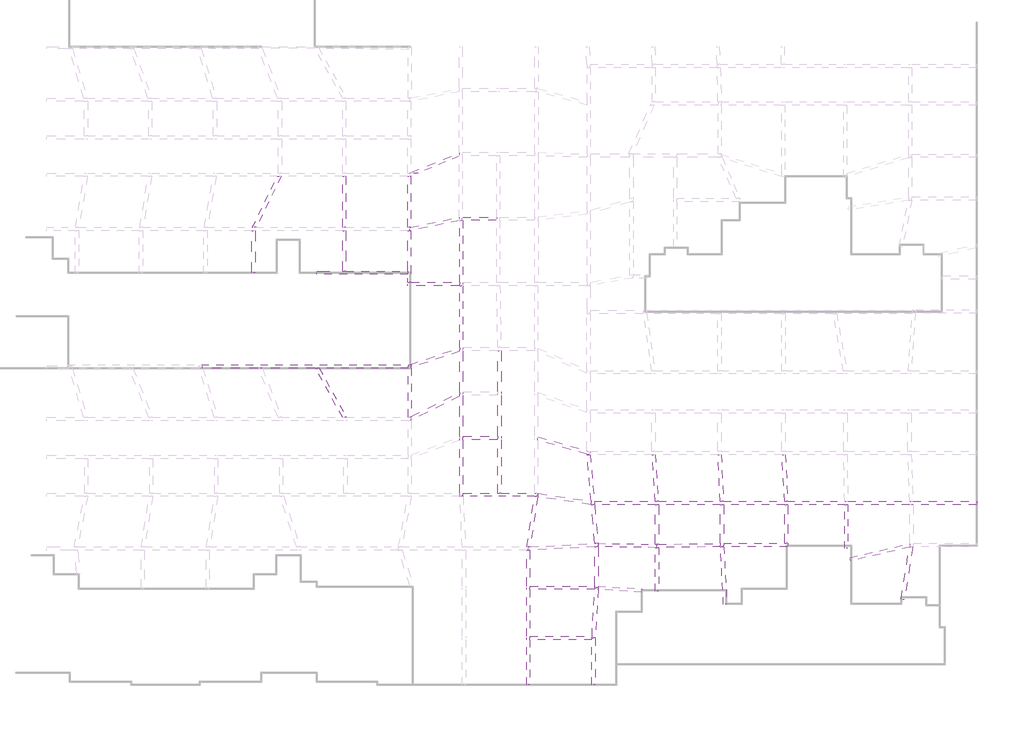
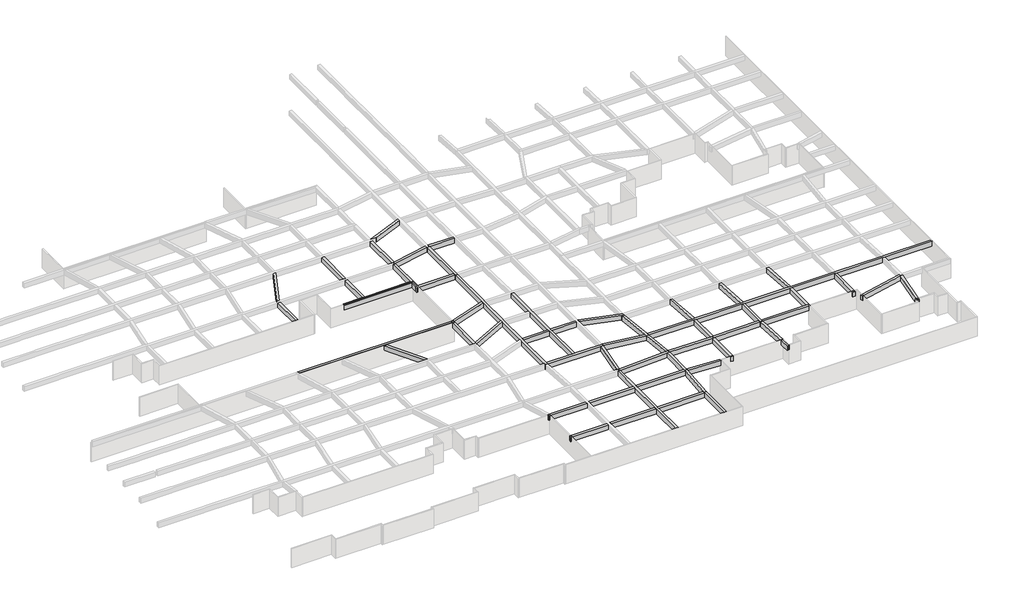
# One storey, part 12 of 45: 49 beams.
"""IFC4 building model written with IfcOpenShell, lengths in millimetres."""

import ifcopenshell
import ifcopenshell.guid

model = None  # the IFC model being written
_history = None  # IfcOwnerHistory: only IFC2X3 demands one
_inside = {}  # id of a spatial element -> (the spatial element, [elements in it])
_under = {}  # id of a project, library or spatial element -> (it, [spatial elements below it])
_declared = {}  # id of a project -> (the project, [libraries it declares])
_typed = {}  # id of a type object -> (the type object, [elements of that type])
_made_of = {}  # id of a material, layer set ... -> (it, [elements and type objects made of it])


def new_model(schema):
    """Start an empty IFC model of exactly this schema.

    Asked for "IFC4X3", IfcOpenShell would pick the latest addendum, in which some entities
    have other attributes; the version numbers below select the first issue.
    IFC2X3 requires an IfcOwnerHistory on every rooted entity: one is made here for all.
    """
    global model, _history
    if schema == "IFC4X3":
        model = ifcopenshell.file(schema_version=(4, 3, 0, 0))
    else:
        model = ifcopenshell.file(schema=schema)
    _inside.clear()
    _under.clear()
    _declared.clear()
    _typed.clear()
    _made_of.clear()
    _history = None
    if model.schema == "IFC2X3":
        org = make("IfcOrganization", Name="unknown")
        user = make(
            "IfcPersonAndOrganization",
            ThePerson=make("IfcPerson", FamilyName="unknown"),
            TheOrganization=org,
        )
        app = make(
            "IfcApplication",
            ApplicationDeveloper=org,
            Version="unknown",
            ApplicationFullName="unknown",
            ApplicationIdentifier="unknown",
        )
        _history = make(
            "IfcOwnerHistory",
            OwningUser=user,
            OwningApplication=app,
            ChangeAction="ADDED",
            CreationDate=0,
        )
    return model


def make(cls, **values):
    """One entity of the class cls with the attributes given. An attribute that is None is left unset."""
    return model.create_entity(
        cls, **{name: value for name, value in values.items() if value is not None}
    )


def rooted(cls, **values):
    """An entity with a GlobalId (a new one), such as an element, a storey or a relation."""
    return make(cls, GlobalId=ifcopenshell.guid.new(), OwnerHistory=_history, **values)


def si_unit(unit_type, name, prefix=None):
    """IfcSIUnit, for example si_unit("LENGTHUNIT", "METRE", prefix="MILLI")."""
    return make("IfcSIUnit", UnitType=unit_type, Prefix=prefix, Name=name)


def assignment(units):
    """IfcUnitAssignment: the units of a project."""
    return None if units is None else make("IfcUnitAssignment", Units=units)


def point(xyz):
    """IfcCartesianPoint."""
    return None if xyz is None else make("IfcCartesianPoint", Coordinates=xyz)


def direction(xyz):
    """IfcDirection."""
    return None if xyz is None else make("IfcDirection", DirectionRatios=xyz)


def frame(location, z_axis=None, x_axis=None):
    """IfcAxis2Placement3D, a coordinate frame: its origin and axes. An axis left out is left unset."""
    return make(
        "IfcAxis2Placement3D",
        Location=point(location),
        Axis=direction(z_axis),
        RefDirection=direction(x_axis),
    )


def origin():
    """The frame at (0, 0, 0) with its axes left unset."""
    return frame((0.0, 0.0, 0.0))


def place(relative_to, where):
    """IfcLocalPlacement: puts the frame where relative to a parent placement (None: the world)."""
    return make(
        "IfcLocalPlacement", PlacementRelTo=relative_to, RelativePlacement=where
    )


def context(
    kind, dimensions, precision=None, world=None, true_north=None, identifier=None
):
    """IfcGeometricRepresentationContext, for example the 3D "Model" context."""
    return make(
        "IfcGeometricRepresentationContext",
        ContextIdentifier=identifier,
        ContextType=kind,
        CoordinateSpaceDimension=dimensions,
        Precision=precision,
        WorldCoordinateSystem=world,
        TrueNorth=true_north,
    )


def project(units=None, contexts=None):
    """IfcProject with its units and contexts."""
    return rooted(
        "IfcProject",
        Name="project",
        RepresentationContexts=contexts,
        UnitsInContext=assignment(units),
    )


def spatial(cls, under=None, at=None, **own):
    """A site, building, storey or space (cls), placed at a placement, below another one or the project."""
    s = rooted(cls, ObjectPlacement=at, **own)
    if under is not None:
        _under.setdefault(under.id(), (under, []))[1].append(s)
    return s


def polyline(points):
    """IfcPolyline through the points."""
    return make("IfcPolyline", Points=[point(p) for p in points])


def outline(outer, holes=None, kind="AREA"):
    """IfcArbitraryClosedProfileDef: a profile drawn as a closed curve; with holes, ...WithVoids."""
    if holes is None:
        return make("IfcArbitraryClosedProfileDef", ProfileType=kind, OuterCurve=outer)
    return make(
        "IfcArbitraryProfileDefWithVoids",
        ProfileType=kind,
        OuterCurve=outer,
        InnerCurves=holes,
    )


def extrude(swept, where, along, depth):
    """IfcExtrudedAreaSolid: the profile swept, set in the frame where, extruded along a direction by depth."""
    return make(
        "IfcExtrudedAreaSolid",
        SweptArea=swept,
        Position=where,
        ExtrudedDirection=direction(along),
        Depth=depth,
    )


def faces_of(points, faces, orient=None, outer=None):
    """IfcFace entities. A face is a list of loops; a loop is a list of indices into points, from 0.

    orient and outer hold one flag for each loop. By default every Orientation is true, the
    first loop of a face is its IfcFaceOuterBound and the others are IfcFaceBound.
    """
    made = []
    for i, loops in enumerate(faces):
        bounds = []
        for j, loop in enumerate(loops):
            is_outer = j == 0 if outer is None else outer[i][j]
            bounds.append(
                make(
                    "IfcFaceOuterBound" if is_outer else "IfcFaceBound",
                    Bound=make("IfcPolyLoop", Polygon=[points[k] for k in loop]),
                    Orientation=True if orient is None else orient[i][j],
                )
            )
        made.append(make("IfcFace", Bounds=bounds))
    return made


def faceted_brep(points, faces, orient=None, outer=None, voids=None):
    """IfcFacetedBrep: a solid bounded by flat faces; with voids (closed shells), ...WithVoids."""
    shared = [point(p) for p in points]
    hull = make("IfcClosedShell", CfsFaces=faces_of(shared, faces, orient, outer))
    if voids is None:
        return make("IfcFacetedBrep", Outer=hull)
    return make(
        "IfcFacetedBrepWithVoids",
        Outer=hull,
        Voids=[
            make(cls, CfsFaces=faces_of(shared, fs, o, b)) for cls, fs, o, b in voids
        ],
    )


def shape(context_of_items, identifier, shape_type, items):
    """IfcShapeRepresentation: the items that make up one representation, for example the "Body"."""
    return make(
        "IfcShapeRepresentation",
        ContextOfItems=context_of_items,
        RepresentationIdentifier=identifier,
        RepresentationType=shape_type,
        Items=items,
    )


def made_of(thing, what):
    """Note that an element or type object is made of a material, layer set ...; save() writes the relation."""
    if what is not None:
        _made_of.setdefault(what.id(), (what, []))[1].append(thing)
    return thing


def element(
    cls,
    number,
    at=None,
    inside=None,
    cuts=None,
    type_object=None,
    material=None,
    context=None,
    identifier="Body",
    shape_type=None,
    held_by="IfcProductDefinitionShape",
    body=None,
    shapes=None,
    **own,
):
    """One element of the class cls, such as IfcWall. Its Tag is "e" and its number.

    at: its placement. inside: the storey or other place that contains it. cuts: it is an
    opening in that element (IfcRelVoidsElement). A single representation is given by context,
    identifier, shape_type and body (its items); several are given by shapes. held_by: the class
    of the entity that holds the representations. save() writes the other relations.
    """
    e = rooted(cls, Tag="e%d" % number, ObjectPlacement=at, **own)
    if body is not None:
        shapes = [shape(context, identifier, shape_type, body)]
    if shapes is not None:
        e.Representation = make(held_by, Representations=shapes)
    if inside is not None:
        _inside.setdefault(inside.id(), (inside, []))[1].append(e)
    if cuts is not None:
        rooted(
            "IfcRelVoidsElement", RelatingBuildingElement=cuts, RelatedOpeningElement=e
        )
    if type_object is not None:
        _typed.setdefault(type_object.id(), (type_object, []))[1].append(e)
    return made_of(e, material)


def aggregate(whole, parts):
    """IfcRelAggregates: a whole, such as a stair, and the parts it consists of."""
    return rooted("IfcRelAggregates", RelatingObject=whole, RelatedObjects=parts)


def save(model, path):
    """Write the relations noted so far, then the file.

    IfcRelAggregates (storeys below a building ...), IfcRelContainedInSpatialStructure (elements
    in a storey), IfcRelDefinesByType, IfcRelAssociatesMaterial and IfcRelDeclares: one each for
    every whole, place, type object, material and project.
    """
    for whole, parts in _under.values():
        aggregate(whole, parts)
    for where, things in _inside.values():
        rooted(
            "IfcRelContainedInSpatialStructure",
            RelatedElements=things,
            RelatingStructure=where,
        )
    for kind, things in _typed.values():
        rooted("IfcRelDefinesByType", RelatedObjects=things, RelatingType=kind)
    for what, things in _made_of.values():
        rooted("IfcRelAssociatesMaterial", RelatedObjects=things, RelatingMaterial=what)
    for by, libraries in _declared.values():
        rooted("IfcRelDeclares", RelatingContext=by, RelatedDefinitions=libraries)
    model.write(path)


model = new_model("IFC4")

# Units and contexts
model_context = context("Model", 3, world=origin())
ifc_project = project(units=[si_unit("LENGTHUNIT", "METRE", prefix="MILLI")], contexts=[model_context])

# Site, building, storey
site = spatial("IfcSite", under=ifc_project)
building = spatial("IfcBuilding", under=site)
storey = spatial("IfcBuildingStorey", under=building, Name="户型图", Elevation=0.0)

# Beams
placement = place(None, origin())
element("IfcBeam", 1, ObjectType="混凝土 - 矩形梁 : KL_beam", at=placement, inside=storey, context=model_context, shape_type="Brep", body=[
    faceted_brep([(-73841.6921627, -136482.7394466, 3300.0), (-73801.0394369, -136882.7394466, 3300.0), (-73674.2267606, -136856.6940178, 3300.0), (-67830.7823984, -135656.5378646, 3300.0), (-67830.7823984, -135248.1884022, 3300.0), (-73674.2267606, -136448.3445554, 3300.0), (-73841.6921627, -136482.7394466, 2500.0), (-67830.7823984, -135248.1884022, 2500.0), (-73674.2267606, -136448.3445554, 2500.0), (-73801.0394369, -136882.7394466, 2500.0), (-67830.7823984, -135656.5378646, 2500.0), (-73674.2267606, -136856.6940178, 2500.0)], [[[0, 1, 2, 3, 4, 5]], [[6, 0, 5, 4, 7, 8]], [[9, 6, 8, 7, 10, 11]], [[1, 9, 11, 10, 3, 2]], [[1, 0, 6, 9]], [[4, 3, 10, 7]]]),
])
element("IfcBeam", 2, ObjectType="混凝土 - 矩形梁 : KL_beam", at=placement, inside=storey, context=model_context, shape_type="Brep", body=[
    faceted_brep([(-73867.4796211, -129869.3244435, 3300.0), (-72799.6927561, -129869.3244435, 3300.0), (-67830.7823984, -127861.7543451, 3300.0), (-67830.7823984, -127430.3404481, 3300.0), (-73674.2267606, -129791.2452196, 3300.0), (-72799.6927561, -129869.3244435, 2500.0), (-67830.7823984, -127861.7543451, 2500.0), (-73867.4796211, -129869.3244435, 2500.0), (-73674.2267606, -129791.2452196, 2500.0), (-67830.7823984, -127430.3404481, 2500.0)], [[[0, 1, 2, 3, 4]], [[1, 5, 6, 2]], [[5, 7, 8, 9, 6]], [[7, 0, 4, 3, 9, 8]], [[1, 0, 7, 5]], [[3, 2, 6, 9]]]),
])
element("IfcBeam", 3, ObjectType="混凝土 - 矩形梁 : KL_beam", at=placement, inside=storey, context=model_context, shape_type="SweptSolid", body=[
    extrude(outline(polyline([(-73841.6921627, -136482.7394466), (-74074.2267606, -136482.7394466), (-74074.2267606, -130269.3244435), (-73789.7274974, -130269.3244435), (-73674.2267606, -130222.6591167), (-73674.2267606, -136448.3445554), (-73841.6921627, -136482.7394466)])), frame((0.0, 0.0, 2500.0), z_axis=(0.0, 0.0, 1.0), x_axis=(1.0, 0.0, 0.0)), (0.0, 0.0, 1.0), 800.0),
])
element("IfcBeam", 4, ObjectType="混凝土 - 矩形梁 : KL_beam", at=placement, inside=storey, context=model_context, shape_type="SweptSolid", body=[
    extrude(outline(polyline([(-81974.2267606, -130269.3244435), (-81574.2267606, -130269.3244435), (-81574.2267606, -136482.7394466), (-81974.2267606, -136482.7394466), (-81974.2267606, -130269.3244435)])), frame((0.0, 0.0, 2500.0), z_axis=(0.0, 0.0, 1.0), x_axis=(1.0, 0.0, 0.0)), (0.0, 0.0, 1.0), 800.0),
])
element("IfcBeam", 5, ObjectType="混凝土 - 矩形梁 : KL_beam", at=placement, inside=storey, context=model_context, shape_type="SweptSolid", body=[
    extrude(outline(polyline([(-89894.2936664, -130269.3244435), (-89449.2528902, -130269.3244435), (-92479.7378735, -136482.7394466), (-92924.7786497, -136482.7394466), (-89894.2936664, -130269.3244435)])), frame((0.0, 0.0, 2500.0), z_axis=(0.0, 0.0, 1.0), x_axis=(1.0, 0.0, 0.0)), (0.0, 0.0, 1.0), 800.0),
])
element("IfcBeam", 6, ObjectType="混凝土 - 矩形梁 : KL_beam", at=placement, inside=storey, context=model_context, shape_type="SweptSolid", body=[
    extrude(outline(polyline([(-92600.0024046, -141982.9420425), (-93000.0024046, -141982.9420425), (-93000.0024046, -136882.7394466), (-92600.0024046, -136882.7394466), (-92600.0024046, -141982.9420425)])), frame((0.0, 0.0, 2500.0), z_axis=(0.0, 0.0, 1.0), x_axis=(1.0, 0.0, 0.0)), (0.0, 0.0, 1.0), 800.0),
])
element("IfcBeam", 7, ObjectType="混凝土 - 矩形梁 : KL_beam", at=placement, inside=storey, context=model_context, shape_type="Brep", body=[
    faceted_brep([(-67430.7823984, -135211.286122, 3300.0), (-67430.7823984, -135574.3838418, 3300.0), (-67610.4560354, -135611.286122, 3300.0), (-67364.0267672, -135611.286122, 3300.0), (-63277.6696197, -135611.286122, 3300.0), (-63277.6696197, -135211.286122, 3300.0), (-67610.4560354, -135611.286122, 2500.0), (-67364.0267672, -135611.286122, 2500.0), (-63277.6696197, -135611.286122, 2500.0), (-67430.7823984, -135574.3838418, 2500.0), (-67430.7823984, -135211.286122, 2500.0), (-63277.6696197, -135211.286122, 2500.0)], [[[0, 1, 2, 3, 4, 5]], [[2, 6, 7, 8, 4, 3]], [[9, 10, 11, 8, 7, 6]], [[10, 0, 5, 11]], [[9, 1, 0, 10]], [[1, 9, 6, 2]], [[5, 4, 8, 11]]]),
])
element("IfcBeam", 8, ObjectType="混凝土 - 矩形梁 : KL_beam", at=placement, inside=storey, context=model_context, shape_type="Brep", body=[
    faceted_brep([(-67764.0267672, -143549.8954633, 3300.0), (-67763.6944245, -143549.8954633, 3300.0), (-67364.0267672, -143549.8954633, 3300.0), (-67364.0267672, -143149.8954633, 3300.0), (-67364.0267672, -135611.286122, 3300.0), (-67610.4560354, -135611.286122, 3300.0), (-67764.0267672, -135642.8272555, 3300.0), (-67764.0267672, -143149.8954633, 3300.0), (-67364.0267672, -143549.8954633, 2500.0), (-67364.0267672, -143149.8954633, 2500.0), (-67364.0267672, -135611.286122, 2500.0), (-67763.6944245, -143549.8954633, 2500.0), (-67764.0267672, -143549.8954633, 2500.0), (-67764.0267672, -143149.8954633, 2500.0), (-67764.0267672, -135642.8272555, 2500.0), (-67610.4560354, -135611.286122, 2500.0)], [[[0, 1, 2, 3, 4, 5, 6, 7]], [[2, 8, 9, 10, 4, 3]], [[8, 11, 12, 13, 14, 15, 10, 9]], [[6, 14, 13, 12, 0, 7]], [[14, 6, 5, 15]], [[5, 4, 10, 15]], [[2, 1, 0, 12, 11, 8]]]),
])
element("IfcBeam", 9, ObjectType="混凝土 - 矩形梁 : KL_beam", at=placement, inside=storey, context=model_context, shape_type="Brep", body=[
    faceted_brep([(-67363.6944245, -143549.8954633, 3300.0), (-67364.0267672, -143549.8954633, 3300.0), (-67763.6944245, -143549.8954633, 3300.0), (-67763.6944245, -151106.0765434, 3300.0), (-67763.6944245, -151528.0229867, 3300.0), (-67763.6944245, -156525.7729118, 3300.0), (-67763.6944245, -156972.1576109, 3300.0), (-67763.6944245, -161910.3096227, 3300.0), (-67763.6944245, -162336.4574801, 3300.0), (-67763.6944245, -168748.040132, 3300.0), (-67763.6944245, -168955.1326476, 3300.0), (-67763.6944245, -169148.040132, 3300.0), (-67763.6944245, -169149.8954633, 3300.0), (-67753.4873378, -169149.8954633, 3300.0), (-67363.6944245, -169149.8954633, 3300.0), (-67363.6944245, -168749.8954633, 3300.0), (-67363.6944245, -162249.8954633, 3300.0), (-67363.6944245, -161849.8954633, 3300.0), (-67363.6944245, -156849.8954633, 3300.0), (-67363.6944245, -156449.8954633, 3300.0), (-67363.6944245, -151449.8954633, 3300.0), (-67363.6944245, -151049.8954633, 3300.0), (-67763.6944245, -143549.8954633, 2500.0), (-67763.6944245, -151106.0765434, 2500.0), (-67763.6944245, -151528.0229867, 2500.0), (-67763.6944245, -156525.7729118, 2500.0), (-67763.6944245, -156972.1576109, 2500.0), (-67763.6944245, -161910.3096227, 2500.0), (-67763.6944245, -162336.4574801, 2500.0), (-67763.6944245, -168748.040132, 2500.0), (-67763.6944245, -168955.1326476, 2500.0), (-67763.6944245, -169148.040132, 2500.0), (-67763.6944245, -169149.8954633, 2500.0), (-67364.0267672, -143549.8954633, 2500.0), (-67363.6944245, -143549.8954633, 2500.0), (-67363.6944245, -151049.8954633, 2500.0), (-67363.6944245, -151449.8954633, 2500.0), (-67363.6944245, -156449.8954633, 2500.0), (-67363.6944245, -156849.8954633, 2500.0), (-67363.6944245, -161849.8954633, 2500.0), (-67363.6944245, -162249.8954633, 2500.0), (-67363.6944245, -168749.8954633, 2500.0), (-67363.6944245, -169149.8954633, 2500.0), (-67753.4873378, -169149.8954633, 2500.0)], [[[0, 1, 2, 3, 4, 5, 6, 7, 8, 9, 10, 11, 12, 13, 14, 15, 16, 17, 18, 19, 20, 21]], [[2, 22, 23, 24, 25, 26, 27, 28, 29, 30, 31, 32, 12, 11, 10, 9, 8, 7, 6, 5, 4, 3]], [[22, 33, 34, 35, 36, 37, 38, 39, 40, 41, 42, 43, 32, 31, 30, 29, 28, 27, 26, 25, 24, 23]], [[14, 42, 41, 40, 39, 38, 37, 36, 35, 34, 0, 21, 20, 19, 18, 17, 16, 15]], [[0, 34, 33, 22, 2, 1]], [[14, 13, 12, 32, 43, 42]]]),
])
element("IfcBeam", 10, ObjectType="混凝土 - 矩形梁 : KL_beam", at=placement, inside=storey, context=model_context, shape_type="Brep", body=[
    faceted_brep([(-58263.6944245, -169149.8954633, 3300.0), (-58263.6944245, -168964.6073199, 3300.0), (-58263.6944245, -168777.3030911, 3300.0), (-58263.6944245, -168749.8954633, 3300.0), (-58663.6944245, -168749.8954633, 3300.0), (-62739.7956089, -168749.8954633, 3300.0), (-63139.7956089, -168749.8954633, 3300.0), (-67363.6944245, -168749.8954633, 3300.0), (-67363.6944245, -169149.8954633, 3300.0), (-67352.9383994, -169149.8954633, 3300.0), (-58695.4543771, -169149.8954633, 3300.0), (-58291.1020523, -169149.8954633, 3300.0), (-58263.6944245, -169149.8954633, 2500.0), (-67363.6944245, -169149.8954633, 2500.0), (-67352.9383994, -169149.8954633, 2500.0), (-58695.4543771, -169149.8954633, 2500.0), (-58291.1020523, -169149.8954633, 2500.0), (-58263.6944245, -168749.8954633, 2500.0), (-58263.6944245, -168777.3030911, 2500.0), (-58263.6944245, -168964.6073199, 2500.0), (-67363.6944245, -168749.8954633, 2500.0), (-63139.7956089, -168749.8954633, 2500.0), (-62739.7956089, -168749.8954633, 2500.0), (-58663.6944245, -168749.8954633, 2500.0)], [[[0, 1, 2, 3, 4, 5, 6, 7, 8, 9, 10, 11]], [[12, 0, 11, 10, 9, 8, 13, 14, 15, 16]], [[17, 18, 19, 12, 16, 15, 14, 13, 20, 21, 22, 23]], [[3, 17, 23, 22, 21, 20, 7, 6, 5, 4]], [[8, 7, 20, 13]], [[3, 2, 1, 0, 12, 19, 18, 17]]]),
])
element("IfcBeam", 11, ObjectType="混凝土 - 矩形梁 : KL_beam", at=placement, inside=storey, context=model_context, shape_type="Brep", body=[
    faceted_brep([(-63139.7956089, -168749.8954633, 2500.0), (-63139.7956089, -168749.8954633, 3300.0), (-63139.7956089, -162249.8954633, 3300.0), (-63139.7956089, -161849.8954633, 3300.0), (-63139.7956089, -156849.8954633, 3300.0), (-63139.7956089, -156449.8954633, 3300.0), (-63139.7956089, -151449.8954633, 3300.0), (-63139.7956089, -151449.8954633, 2500.0), (-63139.7956089, -156449.8954633, 2500.0), (-63139.7956089, -156849.8954633, 2500.0), (-63139.7956089, -161849.8954633, 2500.0), (-63139.7956089, -162249.8954633, 2500.0), (-62739.7956089, -168749.8954633, 3300.0), (-62739.7956089, -168749.8954633, 2500.0), (-62739.7956089, -151449.8954633, 3300.0), (-62739.7956089, -151449.8954633, 2500.0), (-62739.7956089, -162249.8954633, 3300.0), (-62739.7956089, -161849.8954633, 3300.0), (-62739.7956089, -156849.8954633, 3300.0), (-62739.7956089, -156449.8954633, 3300.0), (-62739.7956089, -156449.8954633, 2500.0), (-62739.7956089, -156849.8954633, 2500.0), (-62739.7956089, -161849.8954633, 2500.0), (-62739.7956089, -162249.8954633, 2500.0)], [[[0, 1, 2, 3, 4, 5, 6, 7, 8, 9, 10, 11]], [[12, 1, 0, 13]], [[14, 15, 7, 6]], [[1, 12, 16, 17, 18, 19, 14, 6, 5, 4, 3, 2]], [[13, 0, 11, 10, 9, 8, 7, 15, 20, 21, 22, 23]], [[12, 13, 23, 22, 21, 20, 15, 14, 19, 18, 17, 16]]]),
])
element("IfcBeam", 12, ObjectType="混凝土 - 矩形梁 : KL_beam", at=placement, inside=storey, context=model_context, shape_type="Brep", body=[
    faceted_brep([(-52029.6221736, -164102.89588, 3300.0), (-52020.0590892, -164069.5454413, 3300.0), (-51919.3672313, -163718.3912016, 3300.0), (-52319.3672313, -163603.6930473, 3300.0), (-58263.6944245, -161899.1846532, 3300.0), (-58263.6944245, -162315.3044276, 3300.0), (-52306.232201, -164023.579231, 3300.0), (-52145.9289751, -164069.5454413, 3300.0), (-52029.6221736, -164102.89588, 2500.0), (-58263.6944245, -162315.3044276, 2500.0), (-52306.232201, -164023.579231, 2500.0), (-52145.9289751, -164069.5454413, 2500.0), (-51919.3672313, -163718.3912016, 2500.0), (-52020.0590892, -164069.5454413, 2500.0), (-58263.6944245, -161899.1846532, 2500.0), (-52319.3672313, -163603.6930473, 2500.0)], [[[0, 1, 2, 3, 4, 5, 6, 7]], [[8, 0, 7, 6, 5, 9, 10, 11]], [[12, 13, 8, 11, 10, 9, 14, 15]], [[2, 12, 15, 14, 4, 3]], [[5, 4, 14, 9]], [[2, 1, 0, 8, 13, 12]]]),
])
element("IfcBeam", 13, ObjectType="混凝土 - 矩形梁 : KL_beam", at=placement, inside=storey, context=model_context, shape_type="Brep", body=[
    faceted_brep([(-51770.5606479, -170146.3330997, 3300.0), (-51369.0327129, -170146.3330997, 3300.0), (-51404.0281783, -169746.3330997, 3300.0), (-51900.6827437, -164069.5454413, 3300.0), (-51919.3672313, -164069.5454413, 3300.0), (-52020.0590892, -164069.5454413, 3300.0), (-52029.6221736, -164102.89588, 3300.0), (-52145.9289751, -164069.5454413, 3300.0), (-52302.2106787, -164069.5454413, 3300.0), (-51806.7747625, -169732.4038754, 3300.0), (-51770.9347036, -170142.0576241, 3300.0), (-52302.2106787, -164069.5454413, 2500.0), (-51806.7747625, -169732.4038754, 2500.0), (-51770.9347036, -170142.0576241, 2500.0), (-51770.5606479, -170146.3330997, 2500.0), (-51369.0327129, -170146.3330997, 2500.0), (-52145.9289751, -164069.5454413, 2500.0), (-52029.6221736, -164102.89588, 2500.0), (-52020.0590892, -164069.5454413, 2500.0), (-51919.3672313, -164069.5454413, 2500.0), (-51900.6827437, -164069.5454413, 2500.0), (-51404.0281783, -169746.3330997, 2500.0)], [[[0, 1, 2, 3, 4, 5, 6, 7, 8, 9, 10]], [[8, 11, 12, 13, 14, 0, 10, 9]], [[15, 14, 13, 12, 11, 16, 17, 18, 19, 20, 21]], [[20, 3, 2, 1, 15, 21]], [[11, 8, 7, 16]], [[6, 17, 16, 7]], [[17, 6, 5, 18]], [[3, 20, 19, 18, 5, 4]], [[1, 0, 14, 15]]]),
])
element("IfcBeam", 14, ObjectType="混凝土 - 矩形梁 : KL_beam", at=placement, inside=storey, context=model_context, shape_type="Brep", body=[
    faceted_brep([(-4940.9080348, -169746.3330997, 3300.0), (-4940.9080348, -170146.3330997, 3300.0), (-4940.9080348, -170146.3330997, 2500.0), (-4940.9080348, -169746.3330997, 2500.0), (-12714.0233753, -169746.3330997, 3300.0), (-13114.267193, -169746.3330997, 3300.0), (-20616.7570555, -169746.3330997, 3300.0), (-21016.8179867, -169746.3330997, 3300.0), (-27911.1033716, -169746.3330997, 3300.0), (-28311.65231, -169746.3330997, 3300.0), (-35711.0778615, -169746.3330997, 3300.0), (-36111.6267999, -169746.3330997, 3300.0), (-43613.8318582, -169746.3330997, 3300.0), (-44014.7807223, -169746.3330997, 3300.0), (-51404.0281783, -169746.3330997, 3300.0), (-51369.0327129, -170146.3330997, 3300.0), (-44000.5141412, -170146.3330997, 3300.0), (-43600.5141412, -170146.3330997, 3300.0), (-36100.8707749, -170146.3330997, 3300.0), (-35700.8707749, -170146.3330997, 3300.0), (-28300.8996112, -170146.3330997, 3300.0), (-27900.8996112, -170146.3330997, 3300.0), (-21013.2940066, -170146.3330997, 3300.0), (-20613.2940066, -170146.3330997, 3300.0), (-13107.1611302, -170146.3330997, 3300.0), (-12707.1611302, -170146.3330997, 3300.0), (-51369.0327129, -170146.3330997, 2500.0), (-44000.5141412, -170146.3330997, 2500.0), (-43600.5141412, -170146.3330997, 2500.0), (-36100.8707749, -170146.3330997, 2500.0), (-35700.8707749, -170146.3330997, 2500.0), (-28300.8996112, -170146.3330997, 2500.0), (-27900.8996112, -170146.3330997, 2500.0), (-21013.2940066, -170146.3330997, 2500.0), (-20613.2940066, -170146.3330997, 2500.0), (-13107.1611302, -170146.3330997, 2500.0), (-12707.1611302, -170146.3330997, 2500.0), (-51404.0281783, -169746.3330997, 2500.0), (-44014.7807223, -169746.3330997, 2500.0), (-43613.8318582, -169746.3330997, 2500.0), (-36111.6267999, -169746.3330997, 2500.0), (-35711.0778615, -169746.3330997, 2500.0), (-28311.65231, -169746.3330997, 2500.0), (-27911.1033716, -169746.3330997, 2500.0), (-21016.8179867, -169746.3330997, 2500.0), (-20616.7570555, -169746.3330997, 2500.0), (-13114.267193, -169746.3330997, 2500.0), (-12714.0233753, -169746.3330997, 2500.0)], [[[0, 1, 2, 3]], [[1, 0, 4, 5, 6, 7, 8, 9, 10, 11, 12, 13, 14, 15, 16, 17, 18, 19, 20, 21, 22, 23, 24, 25]], [[2, 1, 25, 24, 23, 22, 21, 20, 19, 18, 17, 16, 15, 26, 27, 28, 29, 30, 31, 32, 33, 34, 35, 36]], [[3, 2, 36, 35, 34, 33, 32, 31, 30, 29, 28, 27, 26, 37, 38, 39, 40, 41, 42, 43, 44, 45, 46, 47]], [[0, 3, 47, 46, 45, 44, 43, 42, 41, 40, 39, 38, 37, 14, 13, 12, 11, 10, 9, 8, 7, 6, 5, 4]], [[15, 14, 37, 26]]]),
])
element("IfcBeam", 15, ObjectType="混凝土 - 矩形梁 : KL_beam", at=placement, inside=storey, context=model_context, shape_type="SweptSolid", body=[
    extrude(outline(polyline([(-36409.1346345, -164069.5454413), (-36008.5856961, -164069.5454413), (-35711.0778615, -169746.3330997), (-36111.6267999, -169746.3330997), (-36409.1346345, -164069.5454413)])), frame((0.0, 0.0, 2500.0), z_axis=(0.0, 0.0, 1.0), x_axis=(1.0, 0.0, 0.0)), (0.0, 0.0, 1.0), 800.0),
])
element("IfcBeam", 16, ObjectType="混凝土 - 矩形梁 : KL_beam", at=placement, inside=storey, context=model_context, shape_type="Brep", body=[
    faceted_brep([(-36100.8707749, -175246.3330997, 3300.0), (-35899.5132097, -175246.3330997, 3300.0), (-35700.8707749, -175246.3330997, 3300.0), (-35700.8707749, -174846.3330997, 3300.0), (-35700.8707749, -170146.3330997, 3300.0), (-36100.8707749, -170146.3330997, 3300.0), (-36100.8707749, -174849.0299244, 3300.0), (-36100.8707749, -175246.3330997, 2500.0), (-36100.8707749, -170146.3330997, 2500.0), (-36100.8707749, -174849.0299244, 2500.0), (-35700.8707749, -175246.3330997, 2500.0), (-35899.5132097, -175246.3330997, 2500.0), (-35700.8707749, -170146.3330997, 2500.0), (-35700.8707749, -174846.3330997, 2500.0)], [[[0, 1, 2, 3, 4, 5, 6]], [[7, 0, 6, 5, 8, 9]], [[10, 11, 7, 9, 8, 12, 13]], [[2, 10, 13, 12, 4, 3]], [[5, 4, 12, 8]], [[2, 1, 0, 7, 11, 10]]]),
])
element("IfcBeam", 17, ObjectType="混凝土 - 矩形梁 : KL_beam", at=placement, inside=storey, context=model_context, shape_type="SweptSolid", body=[
    extrude(outline(polyline([(-28609.1601446, -164069.5454413), (-28208.6112062, -164069.5454413), (-27911.1033716, -169746.3330997), (-28311.65231, -169746.3330997), (-28609.1601446, -164069.5454413)])), frame((0.0, 0.0, 2500.0), z_axis=(0.0, 0.0, 1.0), x_axis=(1.0, 0.0, 0.0)), (0.0, 0.0, 1.0), 800.0),
])
element("IfcBeam", 18, ObjectType="混凝土 - 矩形梁 : KL_beam", at=placement, inside=storey, context=model_context, shape_type="Brep", body=[
    faceted_brep([(-27900.8996112, -175246.3330997, 3300.0), (-27900.8996112, -174846.3330997, 3300.0), (-28300.8996112, -174846.3330997, 3300.0), (-35700.8707749, -174846.3330997, 3300.0), (-35700.8707749, -175246.3330997, 3300.0), (-35689.629168, -175246.3330997, 3300.0), (-27900.8996112, -175246.3330997, 2500.0), (-35700.8707749, -175246.3330997, 2500.0), (-35689.629168, -175246.3330997, 2500.0), (-27900.8996112, -174846.3330997, 2500.0), (-35700.8707749, -174846.3330997, 2500.0), (-28300.8996112, -174846.3330997, 2500.0)], [[[0, 1, 2, 3, 4, 5]], [[6, 0, 5, 4, 7, 8]], [[9, 6, 8, 7, 10, 11]], [[1, 9, 11, 10, 3, 2]], [[4, 3, 10, 7]], [[1, 0, 6, 9]]]),
])
element("IfcBeam", 19, ObjectType="混凝土 - 矩形梁 : KL_beam", at=placement, inside=storey, context=model_context, shape_type="SweptSolid", body=[
    extrude(outline(polyline([(-27900.8996112, -174846.3330997), (-28300.8996112, -174846.3330997), (-28300.8996112, -170146.3330997), (-27900.8996112, -170146.3330997), (-27900.8996112, -174846.3330997)])), frame((0.0, 0.0, 2500.0), z_axis=(0.0, 0.0, 1.0), x_axis=(1.0, 0.0, 0.0)), (0.0, 0.0, 1.0), 800.0),
])
element("IfcBeam", 20, ObjectType="混凝土 - 矩形梁 : KL_beam", at=placement, inside=storey, context=model_context, shape_type="SweptSolid", body=[
    extrude(outline(polyline([(-20613.2940066, -175446.4047579), (-21013.2940066, -175446.4047579), (-21013.2940066, -170146.3330997), (-20613.2940066, -170146.3330997), (-20613.2940066, -175446.4047579)])), frame((0.0, 0.0, 2500.0), z_axis=(0.0, 0.0, 1.0), x_axis=(1.0, 0.0, 0.0)), (0.0, 0.0, 1.0), 800.0),
])
element("IfcBeam", 21, ObjectType="混凝土 - 矩形梁 : KL_beam", at=placement, inside=storey, context=model_context, shape_type="Brep", body=[
    faceted_brep([(-43800.2460734, -175353.5956365, 3300.0), (-43600.1428301, -175350.8789795, 3300.0), (-36090.0425443, -175248.9197787, 3300.0), (-35899.5132097, -175246.3330997, 3300.0), (-36100.8707749, -175246.3330997, 3300.0), (-36100.8707749, -174849.0299244, 3300.0), (-43600.5141412, -174950.8471592, 3300.0), (-43800.0395867, -174953.5559719, 3300.0), (-36100.8707749, -174849.0299244, 2500.0), (-43600.5141412, -174950.8471592, 2500.0), (-43800.0395867, -174953.5559719, 2500.0), (-36100.8707749, -175246.3330997, 2500.0), (-35899.5132097, -175246.3330997, 2500.0), (-36090.0425443, -175248.9197787, 2500.0), (-43600.1428301, -175350.8789795, 2500.0), (-43800.2460734, -175353.5956365, 2500.0)], [[[0, 1, 2, 3, 4, 5, 6, 7]], [[7, 6, 5, 8, 9, 10]], [[10, 9, 8, 11, 12, 13, 14, 15]], [[3, 2, 1, 0, 15, 14, 13, 12]], [[4, 11, 8, 5]], [[11, 4, 3, 12]], [[0, 7, 10, 15]]]),
])
element("IfcBeam", 22, ObjectType="混凝土 - 矩形梁 : KL_beam", at=placement, inside=storey, context=model_context, shape_type="Brep", body=[
    faceted_brep([(-59434.9645519, -175280.7215365, 3300.0), (-59424.4901833, -175680.7215365, 3300.0), (-59229.7273676, -175670.5144499, 3300.0), (-51349.1150073, -175257.5090567, 3300.0), (-50949.1150073, -175236.545945, 3300.0), (-50937.7619715, -175235.9509576, 3300.0), (-50949.1150073, -175019.3221294, 3300.0), (-50958.0419428, -174848.9860526, 3300.0), (-50958.696354, -174836.4991437, 3300.0), (-51358.3916515, -174857.4462866, 3300.0), (-59196.1158349, -175268.2040057, 3300.0), (-59434.9645519, -175280.7215365, 2500.0), (-50958.696354, -174836.4991437, 2500.0), (-51358.3916515, -174857.4462866, 2500.0), (-59196.1158349, -175268.2040057, 2500.0), (-59424.4901833, -175680.7215365, 2500.0), (-50958.0419428, -174848.9860526, 2500.0), (-50949.1150073, -175019.3221294, 2500.0), (-50937.7619715, -175235.9509576, 2500.0), (-50949.1150073, -175236.545945, 2500.0), (-51349.1150073, -175257.5090567, 2500.0), (-59229.7273676, -175670.5144499, 2500.0)], [[[0, 1, 2, 3, 4, 5, 6, 7, 8, 9, 10]], [[11, 0, 10, 9, 8, 12, 13, 14]], [[15, 11, 14, 13, 12, 16, 17, 18, 19, 20, 21]], [[1, 15, 21, 20, 19, 18, 5, 4, 3, 2]], [[5, 18, 17, 16, 12, 8, 7, 6]], [[1, 0, 11, 15]]]),
])
element("IfcBeam", 23, ObjectType="混凝土 - 矩形梁 : KL_beam", at=placement, inside=storey, context=model_context, shape_type="Brep", body=[
    faceted_brep([(-59229.7273676, -192027.8669315, 3300.0), (-59629.7273676, -192027.8669315, 3300.0), (-59629.7273676, -192027.8669315, 2500.0), (-59229.7273676, -192027.8669315, 2500.0), (-59229.7273676, -186528.0123265, 3300.0), (-59229.7273676, -186128.0123265, 3300.0), (-59229.7273676, -180443.730522, 3300.0), (-59229.7273676, -180043.730522, 3300.0), (-59229.7273676, -175670.5144499, 3300.0), (-59424.4901833, -175680.7215365, 3300.0), (-59629.7273676, -175680.7215365, 3300.0), (-59629.7273676, -180043.730522, 3300.0), (-59629.7273676, -180443.730522, 3300.0), (-59629.7273676, -186128.0123265, 3300.0), (-59629.7273676, -186528.0123265, 3300.0), (-59629.7273676, -175680.7215365, 2500.0), (-59629.7273676, -180043.730522, 2500.0), (-59629.7273676, -180443.730522, 2500.0), (-59629.7273676, -186128.0123265, 2500.0), (-59629.7273676, -186528.0123265, 2500.0), (-59424.4901833, -175680.7215365, 2500.0), (-59229.7273676, -175670.5144499, 2500.0), (-59229.7273676, -180043.730522, 2500.0), (-59229.7273676, -180443.730522, 2500.0), (-59229.7273676, -186128.0123265, 2500.0), (-59229.7273676, -186528.0123265, 2500.0)], [[[0, 1, 2, 3]], [[1, 0, 4, 5, 6, 7, 8, 9, 10, 11, 12, 13, 14]], [[2, 1, 14, 13, 12, 11, 10, 15, 16, 17, 18, 19]], [[3, 2, 19, 18, 17, 16, 15, 20, 21, 22, 23, 24, 25]], [[0, 3, 25, 24, 23, 22, 21, 8, 7, 6, 5, 4]], [[9, 8, 21, 20]], [[10, 9, 20, 15]]]),
])
element("IfcBeam", 24, ObjectType="混凝土 - 矩形梁 : KL_beam", at=placement, inside=storey, context=model_context, shape_type="Brep", body=[
    faceted_brep([(-51700.5216564, -192028.0123265, 3300.0), (-51700.5216564, -192028.0123265, 2500.0), (-51300.5216564, -192028.0123265, 2500.0), (-51300.5216564, -192028.0123265, 3300.0), (-51300.5216564, -186333.7831438, 3300.0), (-51700.5216564, -186322.2415091, 3300.0), (-51700.5216564, -186528.0123265, 3300.0), (-51300.5216564, -186333.7831438, 2500.0), (-51700.5216564, -186322.2415091, 2500.0), (-51700.5216564, -186528.0123265, 2500.0)], [[[0, 1, 2, 3]], [[4, 5, 6, 0, 3]], [[7, 4, 3, 2]], [[8, 7, 2, 1, 9]], [[5, 8, 9, 1, 0, 6]], [[5, 4, 7, 8]]]),
])
element("IfcBeam", 25, ObjectType="混凝土 - 矩形梁 : KL_beam", at=placement, inside=storey, context=model_context, shape_type="Brep", body=[
    faceted_brep([(-51300.5216564, -186333.7831438, 3300.0), (-50960.9810787, -180454.9298094, 3300.0), (-50949.1150073, -180249.4789789, 3300.0), (-51349.1150073, -180237.9373442, 3300.0), (-51361.0008515, -180443.730522, 3300.0), (-51689.3037054, -186128.0123265, 3300.0), (-51700.5216564, -186322.2415091, 3300.0), (-51349.1150073, -180237.9373442, 2500.0), (-51361.0008515, -180443.730522, 2500.0), (-51689.3037054, -186128.0123265, 2500.0), (-51700.5216564, -186322.2415091, 2500.0), (-50949.1150073, -180249.4789789, 2500.0), (-50960.9810787, -180454.9298094, 2500.0), (-51300.5216564, -186333.7831438, 2500.0)], [[[0, 1, 2, 3, 4, 5, 6]], [[6, 5, 4, 3, 7, 8, 9, 10]], [[10, 9, 8, 7, 11, 12, 13]], [[2, 1, 0, 13, 12, 11]], [[0, 6, 10, 13]], [[2, 11, 7, 3]]]),
])
element("IfcBeam", 26, ObjectType="混凝土 - 矩形梁 : KL_beam", at=placement, inside=storey, context=model_context, shape_type="Brep", body=[
    faceted_brep([(-50949.1150073, -174849.1164646, 3300.0), (-50957.6033304, -174848.9924602, 3300.0), (-50958.0419428, -174848.9860526, 3300.0), (-50949.1150073, -175019.3221294, 3300.0), (-50949.1150073, -174946.0144374, 3300.0), (-50949.1150073, -174849.1164646, 2500.0), (-50949.1150073, -175019.3221294, 2500.0), (-50949.1150073, -174946.0144374, 2500.0), (-50958.0419428, -174848.9860526, 2500.0), (-50957.6033304, -174848.9924602, 2500.0)], [[[0, 1, 2, 3, 4]], [[5, 0, 4, 3, 6, 7]], [[8, 9, 5, 7, 6]], [[0, 5, 9, 8, 2, 1]], [[3, 2, 8, 6]]]),
    faceted_brep([(-51349.1150073, -180237.9373442, 2500.0), (-51349.1150073, -180237.9373442, 3300.0), (-51349.1150073, -180043.730522, 3300.0), (-51349.1150073, -175257.5090567, 3300.0), (-51349.1150073, -175257.5090567, 2500.0), (-51349.1150073, -180043.730522, 2500.0), (-50949.1150073, -180249.4789789, 2500.0), (-50949.1150073, -180249.4789789, 3300.0), (-50949.1150073, -175236.545945, 3300.0), (-50949.1150073, -175236.545945, 2500.0), (-50949.1150073, -180054.9485476, 3300.0), (-50949.1150073, -175249.1591458, 3300.0), (-50949.1150073, -180054.9485476, 2500.0), (-50949.1150073, -175249.1591458, 2500.0)], [[[0, 1, 2, 3, 4, 5]], [[1, 0, 6, 7]], [[3, 8, 9, 4]], [[1, 7, 10, 11, 8, 3, 2]], [[7, 6, 12, 13, 9, 8, 11, 10]], [[6, 0, 5, 4, 9, 13, 12]]]),
])
element("IfcBeam", 27, ObjectType="混凝土 - 矩形梁 : KL_beam", at=placement, inside=storey, context=model_context, shape_type="SweptSolid", body=[
    extrude(outline(polyline([(-73600.5216564, -186528.0123265), (-73600.5216564, -186128.0123265), (-67421.4283331, -186128.0123265), (-67421.4283331, -186528.0123265), (-73600.5216564, -186528.0123265)])), frame((0.0, 0.0, 2500.0), z_axis=(0.0, 0.0, 1.0), x_axis=(1.0, 0.0, 0.0)), (0.0, 0.0, 1.0), 800.0),
    extrude(outline(polyline([(-51700.5216564, -186322.2415091), (-51700.5216564, -186528.0123265), (-59229.7273676, -186528.0123265), (-59229.7273676, -186128.0123265), (-51689.3037054, -186128.0123265), (-51700.5216564, -186322.2415091)])), frame((0.0, 0.0, 2500.0), z_axis=(0.0, 0.0, 1.0), x_axis=(1.0, 0.0, 0.0)), (0.0, 0.0, 1.0), 800.0),
    extrude(outline(polyline([(-67021.4283331, -186528.0123265), (-67021.4283331, -186128.0123265), (-59629.7273676, -186128.0123265), (-59629.7273676, -186528.0123265), (-67021.4283331, -186528.0123265)])), frame((0.0, 0.0, 2500.0), z_axis=(0.0, 0.0, 1.0), x_axis=(1.0, 0.0, 0.0)), (0.0, 0.0, 1.0), 800.0),
])
element("IfcBeam", 28, ObjectType="混凝土 - 矩形梁 : KL_beam", at=placement, inside=storey, context=model_context, shape_type="Brep", body=[
    faceted_brep([(-58263.6944245, -168777.3030911, 3300.0), (-58263.6944245, -168964.6073199, 3300.0), (-58236.581804, -168781.3135615, 3300.0), (-58263.6944245, -168964.6073199, 2500.0), (-58236.581804, -168781.3135615, 2500.0), (-58263.6944245, -168777.3030911, 2500.0)], [[[0, 1, 2]], [[1, 3, 4, 2]], [[3, 5, 4]], [[1, 0, 5, 3]], [[2, 4, 5, 0]]]),
    faceted_brep([(-58695.4543771, -169149.8954633, 3300.0), (-58695.4543771, -169149.8954633, 2500.0), (-59602.3197398, -175280.7215365, 2500.0), (-59602.3197398, -175280.7215365, 3300.0), (-58291.1020523, -169149.8954633, 3300.0), (-58291.1020523, -169149.8954633, 2500.0), (-58663.6944245, -169149.8954633, 2500.0), (-58663.6944245, -169149.8954633, 3300.0), (-59434.9645519, -175280.7215365, 3300.0), (-59434.9645519, -175280.7215365, 2500.0), (-59229.7273676, -175269.9655115, 2500.0), (-59196.1158349, -175268.2040057, 2500.0), (-59196.1158349, -175268.2040057, 3300.0), (-59229.7273676, -175269.9655115, 3300.0), (-58295.1125227, -169177.0080838, 3300.0), (-58295.1125227, -169177.0080838, 2500.0)], [[[0, 1, 2, 3]], [[4, 5, 6, 1, 0, 7]], [[8, 9, 10, 11, 12, 13]], [[3, 2, 9, 8]], [[12, 14, 4, 7, 0, 3, 8, 13]], [[5, 4, 14, 12, 11, 15]], [[5, 15, 11, 10, 9, 2, 1, 6]]]),
])
element("IfcBeam", 29, ObjectType="混凝土 - 矩形梁 : KL_beam", at=placement, inside=storey, context=model_context, shape_type="SweptSolid", body=[
    extrude(outline(polyline([(-58291.1020523, -169149.8954633), (-58263.6944245, -169149.8954633), (-58263.6944245, -168964.6073199), (-58236.581804, -168781.3135615), (-51806.7747625, -169732.4038754), (-51770.9347036, -170142.0576241), (-58295.1125227, -169177.0080838), (-58291.1020523, -169149.8954633)])), frame((0.0, 0.0, 2500.0), z_axis=(0.0, 0.0, 1.0), x_axis=(1.0, 0.0, 0.0)), (0.0, 0.0, 1.0), 800.0),
])
element("IfcBeam", 30, ObjectType="混凝土 - 矩形梁 : KL_beam", at=placement, inside=storey, context=model_context, shape_type="Brep", body=[
    faceted_brep([(-51369.0327129, -170146.3330997, 3300.0), (-51770.5606479, -170146.3330997, 3300.0), (-51358.3916515, -174857.4462866, 3300.0), (-51349.1150073, -174856.9601183, 3300.0), (-51144.8793325, -174846.2565801, 3300.0), (-50958.696354, -174836.4991437, 3300.0), (-51770.5606479, -170146.3330997, 2500.0), (-51358.3916515, -174857.4462866, 2500.0), (-51369.0327129, -170146.3330997, 2500.0), (-50958.696354, -174836.4991437, 2500.0), (-51144.8793325, -174846.2565801, 2500.0), (-51349.1150073, -174856.9601183, 2500.0), (-50957.6033304, -174848.9924602, 3300.0), (-50957.6033304, -174848.9924602, 2500.0), (-50958.0419428, -174848.9860526, 2500.0), (-50958.0419428, -174848.9860526, 3300.0)], [[[0, 1, 2, 3, 4, 5]], [[1, 6, 7, 2]], [[6, 8, 9, 10, 11, 7]], [[8, 0, 5, 12, 13, 9]], [[1, 0, 8, 6]], [[9, 5, 4, 3, 2, 7, 11, 10]], [[5, 9, 14, 15]], [[13, 12, 15, 14]], [[12, 5, 15]], [[9, 13, 14]]]),
    faceted_brep([(-50923.8128068, -175235.2199128, 2500.0), (-50923.8128068, -175235.2199128, 3300.0), (-50937.7619715, -175235.9509576, 3300.0), (-50937.7619715, -175235.9509576, 2500.0), (-50949.1150073, -174946.0144374, 3300.0), (-50949.1150073, -175019.3221294, 3300.0), (-50949.1150073, -175019.3221294, 2500.0), (-50949.1150073, -174946.0144374, 2500.0)], [[[0, 1, 2, 3]], [[2, 1, 4, 5]], [[0, 3, 6, 7]], [[4, 7, 6, 5]], [[1, 0, 7, 4]], [[3, 2, 5, 6]]]),
])
element("IfcBeam", 31, ObjectType="混凝土 - 矩形梁 : KL_beam", at=placement, inside=storey, context=model_context, shape_type="Brep", body=[
    faceted_brep([(-43800.2460734, -175353.5956365, 2500.0), (-43800.2460734, -175353.5956365, 3300.0), (-44000.1428301, -175350.6753822, 3300.0), (-50949.1150073, -175249.1591458, 3300.0), (-50949.1150073, -175249.1591458, 2500.0), (-44000.1428301, -175350.6753822, 2500.0), (-43800.0395867, -174953.5559719, 2500.0), (-43800.0395867, -174953.5559719, 3300.0), (-50923.8128068, -175235.2199128, 3300.0), (-50923.8128068, -175235.2199128, 2500.0), (-50937.7619715, -175235.9509576, 2500.0), (-50949.1150073, -175236.545945, 2500.0), (-50949.1150073, -175236.545945, 3300.0), (-50937.7619715, -175235.9509576, 3300.0), (-44000.5141412, -174950.6272765, 3300.0), (-50949.1150073, -174849.1164646, 3300.0), (-50949.1150073, -174946.0144374, 3300.0), (-44000.5141412, -174950.6272765, 2500.0), (-50949.1150073, -174849.1164646, 2500.0), (-50949.1150073, -174946.0144374, 2500.0)], [[[0, 1, 2, 3, 4, 5]], [[1, 0, 6, 7]], [[8, 9, 10, 11, 12, 13]], [[1, 7, 14, 15, 16, 8, 13, 12, 3, 2]], [[7, 6, 17, 18, 15, 14]], [[6, 0, 5, 4, 11, 10, 9, 19, 18, 17]], [[9, 8, 16, 19]], [[16, 15, 18, 19]], [[4, 3, 12, 11]]]),
])
element("IfcBeam", 32, ObjectType="混凝土 - 矩形梁 : KL_beam", at=placement, inside=storey, context=model_context, shape_type="SweptSolid", body=[
    extrude(outline(polyline([(-44000.5141412, -170146.3330997), (-43600.5141412, -170146.3330997), (-43600.5141412, -174950.8471592), (-43800.0395867, -174953.5559719), (-44000.5141412, -174950.6272765), (-44000.5141412, -170146.3330997)])), frame((0.0, 0.0, 2500.0), z_axis=(0.0, 0.0, 1.0), x_axis=(1.0, 0.0, 0.0)), (0.0, 0.0, 1.0), 800.0),
])
element("IfcBeam", 33, ObjectType="混凝土 - 矩形梁 : KL_beam", at=placement, inside=storey, context=model_context, shape_type="SweptSolid", body=[
    extrude(outline(polyline([(-44406.0241434, -164069.5454413), (-44005.0752794, -164069.5454413), (-43613.8318582, -169746.3330997), (-44014.7807223, -169746.3330997), (-44406.0241434, -164069.5454413)])), frame((0.0, 0.0, 2500.0), z_axis=(0.0, 0.0, 1.0), x_axis=(1.0, 0.0, 0.0)), (0.0, 0.0, 1.0), 800.0),
])
element("IfcBeam", 34, ObjectType="混凝土 - 矩形梁 : KL_beam", at=placement, inside=storey, context=model_context, shape_type="SweptSolid", body=[
    extrude(outline(polyline([(-43600.1428301, -180653.5758042), (-44000.1428301, -180653.5758042), (-44000.1428301, -175350.6753822), (-43800.2460734, -175353.5956365), (-43600.1428301, -175350.8789795), (-43600.1428301, -180653.5758042)])), frame((0.0, 0.0, 2500.0), z_axis=(0.0, 0.0, 1.0), x_axis=(1.0, 0.0, 0.0)), (0.0, 0.0, 1.0), 800.0),
])
element("IfcBeam", 35, ObjectType="混凝土 - 矩形梁 : KL_beam", at=placement, inside=storey, context=model_context, shape_type="Brep", body=[
    faceted_brep([(-35323.8404011, -182225.9985587, 3300.0), (-35723.292215, -182246.9329412, 3300.0), (-35723.292215, -182246.9329412, 2500.0), (-35323.8404011, -182225.9985587, 2500.0), (-35689.629168, -175246.3330997, 3300.0), (-35700.8707749, -175246.3330997, 3300.0), (-35899.5132097, -175246.3330997, 3300.0), (-36090.0425443, -175248.9197787, 3300.0), (-36090.0425443, -175248.9197787, 2500.0), (-35899.5132097, -175246.3330997, 2500.0), (-35700.8707749, -175246.3330997, 2500.0), (-35689.629168, -175246.3330997, 2500.0)], [[[0, 1, 2, 3]], [[1, 0, 4, 5, 6, 7]], [[2, 1, 7, 8]], [[3, 2, 8, 9, 10, 11]], [[0, 3, 11, 4]], [[4, 11, 10, 9, 6, 5]], [[7, 6, 9, 8]]]),
])
element("IfcBeam", 36, ObjectType="混凝土 - 矩形梁 : KL_beam", at=placement, inside=storey, context=model_context, shape_type="SweptSolid", body=[
    extrude(outline(polyline([(-45646.7341427, -180361.1942319), (-45669.79821, -180760.5287393), (-50960.9810787, -180454.9298094), (-50949.1150073, -180249.4789789), (-50949.1150073, -180054.9485476), (-45646.7341427, -180361.1942319)])), frame((0.0, 0.0, 2500.0), z_axis=(0.0, 0.0, 1.0), x_axis=(1.0, 0.0, 0.0)), (0.0, 0.0, 1.0), 800.0),
])
element("IfcBeam", 37, ObjectType="混凝土 - 矩形梁 : KL_beam", at=placement, inside=storey, context=model_context, shape_type="SweptSolid", body=[
    extrude(outline(polyline([(-81500.4571592, -159548.040132), (-81957.9933056, -159548.040132), (-85288.7914211, -153549.9677976), (-84831.2552748, -153549.9677976), (-81500.4571592, -159548.040132)])), frame((0.0, 0.0, 2500.0), z_axis=(0.0, 0.0, 1.0), x_axis=(1.0, 0.0, 0.0)), (0.0, 0.0, 1.0), 800.0),
])
element("IfcBeam", 38, ObjectType="混凝土 - 矩形梁 : KL_beam", at=placement, inside=storey, context=model_context, shape_type="Brep", body=[
    faceted_brep([(-73618.1629467, -153149.9677976, 3300.0), (-73850.8435684, -153149.9677976, 3300.0), (-74018.1629467, -153149.9677976, 3300.0), (-74018.1629467, -153549.9677976, 3300.0), (-74018.1629467, -159548.040132, 3300.0), (-73618.1629467, -159548.040132, 3300.0), (-73618.1629467, -159425.7779844, 3300.0), (-73618.1629467, -153493.7867175, 3300.0), (-74018.1629467, -153149.9677976, 2500.0), (-74018.1629467, -153549.9677976, 2500.0), (-74018.1629467, -159548.040132, 2500.0), (-73850.8435684, -153149.9677976, 2500.0), (-73618.1629467, -153149.9677976, 2500.0), (-73618.1629467, -153493.7867175, 2500.0), (-73618.1629467, -159425.7779844, 2500.0), (-73618.1629467, -159548.040132, 2500.0)], [[[0, 1, 2, 3, 4, 5, 6, 7]], [[2, 8, 9, 10, 4, 3]], [[8, 11, 12, 13, 14, 15, 10, 9]], [[12, 0, 7, 6, 5, 15, 14, 13]], [[5, 4, 10, 15]], [[2, 1, 0, 12, 11, 8]]]),
])
element("IfcBeam", 39, ObjectType="混凝土 - 矩形梁 : KL_beam", at=placement, inside=storey, context=model_context, shape_type="Brep", body=[
    faceted_brep([(-99099.3076958, -153149.9677976, 3300.0), (-98977.0154232, -153549.9677976, 3300.0), (-92191.7933969, -153549.9677976, 3300.0), (-91761.4759268, -153549.9677976, 3300.0), (-85288.7914211, -153549.9677976, 3300.0), (-84831.2552748, -153549.9677976, 3300.0), (-74018.1629467, -153549.9677976, 3300.0), (-74018.1629467, -153149.9677976, 3300.0), (-99099.3076958, -153149.9677976, 2500.0), (-74018.1629467, -153149.9677976, 2500.0), (-98977.0154232, -153549.9677976, 2500.0), (-74018.1629467, -153549.9677976, 2500.0), (-84831.2552748, -153549.9677976, 2500.0), (-85288.7914211, -153549.9677976, 2500.0), (-91761.4759268, -153549.9677976, 2500.0), (-92191.7933969, -153549.9677976, 2500.0)], [[[0, 1, 2, 3, 4, 5, 6, 7]], [[8, 0, 7, 9]], [[10, 8, 9, 11, 12, 13, 14, 15]], [[1, 10, 15, 14, 13, 12, 11, 6, 5, 4, 3, 2]], [[1, 0, 8, 10]], [[7, 6, 11, 9]]]),
])
element("IfcBeam", 40, ObjectType="混凝土 - 矩形梁 : KL_beam", at=placement, inside=storey, context=model_context, shape_type="SweptSolid", body=[
    extrude(outline(polyline([(-73618.1629467, -153493.7867175), (-73618.1629467, -153149.9677976), (-73850.8435684, -153149.9677976), (-67763.6944245, -151106.0765434), (-67763.6944245, -151528.0229867), (-73618.1629467, -153493.7867175)])), frame((0.0, 0.0, 2500.0), z_axis=(0.0, 0.0, 1.0), x_axis=(1.0, 0.0, 0.0)), (0.0, 0.0, 1.0), 800.0),
])
element("IfcBeam", 41, ObjectType="混凝土 - 矩形梁 : KL_beam", at=placement, inside=storey, context=model_context, shape_type="Brep", body=[
    faceted_brep([(-67764.0267672, -143149.8954633, 3300.0), (-67764.0267672, -143149.8954633, 2500.0), (-73674.2267606, -143149.8954633, 2500.0), (-74074.2267606, -143149.8954633, 2500.0), (-74074.2267606, -143149.8954633, 3300.0), (-73674.2267606, -143149.8954633, 3300.0), (-67764.0267672, -143549.8954633, 3300.0), (-67764.0267672, -143549.8954633, 2500.0), (-74074.2267606, -143549.8954633, 3300.0), (-74074.2267606, -143549.8954633, 2500.0)], [[[0, 1, 2, 3, 4, 5]], [[0, 6, 7, 1]], [[6, 0, 5, 4, 8]], [[1, 7, 9, 3, 2]], [[7, 6, 8, 9]], [[8, 4, 3, 9]]]),
])
element("IfcBeam", 42, ObjectType="混凝土 - 矩形梁 : KL_beam", at=placement, inside=storey, context=model_context, shape_type="Brep", body=[
    faceted_brep([(-74074.2267606, -143149.8954633, 3300.0), (-73674.2267606, -143149.8954633, 3300.0), (-73674.2267606, -136856.6940178, 3300.0), (-73801.0394369, -136882.7394466, 3300.0), (-74074.2267606, -136882.7394466, 3300.0), (-74074.2267606, -141791.0626808, 3300.0), (-74074.2267606, -142191.0626808, 3300.0), (-74074.2267606, -143149.8954633, 2500.0), (-74074.2267606, -136882.7394466, 2500.0), (-74074.2267606, -141791.0626808, 2500.0), (-74074.2267606, -142191.0626808, 2500.0), (-73674.2267606, -143149.8954633, 2500.0), (-73801.0394369, -136882.7394466, 2500.0), (-73674.2267606, -136856.6940178, 2500.0)], [[[0, 1, 2, 3, 4, 5, 6]], [[7, 0, 6, 5, 4, 8, 9, 10]], [[11, 7, 10, 9, 8, 12, 13]], [[1, 11, 13, 2]], [[1, 0, 7, 11]], [[4, 3, 12, 8]], [[3, 2, 13, 12]]]),
])
element("IfcBeam", 43, ObjectType="混凝土 - 矩形梁 : KL_beam", at=placement, inside=storey, context=model_context, shape_type="SweptSolid", body=[
    extrude(outline(polyline([(-81974.2267606, -136882.7394466), (-81574.2267606, -136882.7394466), (-81574.2267606, -141791.0626808), (-81974.2267606, -141791.0626808), (-81974.2267606, -136882.7394466)])), frame((0.0, 0.0, 2500.0), z_axis=(0.0, 0.0, 1.0), x_axis=(1.0, 0.0, 0.0)), (0.0, 0.0, 1.0), 800.0),
])
element("IfcBeam", 44, ObjectType="混凝土 - 矩形梁 : KL_beam", at=placement, inside=storey, context=model_context, shape_type="Brep", body=[
    faceted_brep([(-85117.3039172, -141791.0626808, 3300.0), (-85117.3039172, -141791.0626808, 2500.0), (-85117.3039172, -142191.0626808, 2500.0), (-85117.3039172, -142191.0626808, 3300.0), (-74074.2267606, -142191.0626808, 3300.0), (-74074.2267606, -141791.0626808, 3300.0), (-81574.2267606, -141791.0626808, 3300.0), (-81974.2267606, -141791.0626808, 3300.0), (-74074.2267606, -142191.0626808, 2500.0), (-81974.2267606, -141791.0626808, 2500.0), (-81574.2267606, -141791.0626808, 2500.0), (-74074.2267606, -141791.0626808, 2500.0)], [[[0, 1, 2, 3]], [[0, 3, 4, 5, 6, 7]], [[3, 2, 8, 4]], [[2, 1, 9, 10, 11, 8]], [[1, 0, 7, 6, 5, 11, 10, 9]], [[5, 4, 8, 11]]]),
])
element("IfcBeam", 45, ObjectType="混凝土 - 矩形梁 : KL_beam", at=placement, inside=storey, context=model_context, shape_type="Brep", body=[
    faceted_brep([(-67421.4283331, -180443.730522, 3300.0), (-67421.4283331, -180043.730522, 3300.0), (-73337.815755, -180043.730522, 3300.0), (-73758.4006447, -180043.730522, 3300.0), (-73628.4327662, -180443.730522, 3300.0), (-67421.4283331, -180043.730522, 2500.0), (-73337.815755, -180043.730522, 2500.0), (-73758.4006447, -180043.730522, 2500.0), (-67421.4283331, -180443.730522, 2500.0), (-73628.4327662, -180443.730522, 2500.0)], [[[0, 1, 2, 3, 4]], [[1, 5, 6, 7, 3, 2]], [[5, 8, 9, 7, 6]], [[8, 0, 4, 9]], [[1, 0, 8, 5]], [[4, 3, 7, 9]]]),
    faceted_brep([(-51349.1150073, -180237.9373442, 3300.0), (-51361.0008515, -180443.730522, 3300.0), (-51361.0008515, -180443.730522, 2500.0), (-51349.1150073, -180237.9373442, 2500.0), (-51349.1150073, -180043.730522, 3300.0), (-51349.1150073, -180043.730522, 2500.0), (-59229.7273676, -180443.730522, 3300.0), (-59229.7273676, -180043.730522, 3300.0), (-59229.7273676, -180043.730522, 2500.0), (-59229.7273676, -180443.730522, 2500.0)], [[[0, 1, 2, 3]], [[4, 0, 3, 5]], [[6, 7, 8, 9]], [[1, 0, 4, 7, 6]], [[4, 5, 8, 7]], [[3, 2, 9, 8, 5]], [[2, 1, 6, 9]]]),
    faceted_brep([(-67021.4283331, -180443.730522, 3300.0), (-67021.4283331, -180043.730522, 3300.0), (-67021.4283331, -180043.730522, 2500.0), (-67021.4283331, -180443.730522, 2500.0), (-59629.7273676, -180443.730522, 3300.0), (-59629.7273676, -180043.730522, 3300.0), (-59629.7273676, -180043.730522, 2500.0), (-59629.7273676, -180443.730522, 2500.0)], [[[0, 1, 2, 3]], [[1, 0, 4, 5]], [[2, 1, 5, 6]], [[3, 2, 6, 7]], [[0, 3, 7, 4]], [[5, 4, 7, 6]]]),
])
element("IfcBeam", 46, ObjectType="混凝土 - 矩形梁 : KL_beam", at=placement, inside=storey, context=model_context, shape_type="SweptSolid", body=[
    extrude(outline(polyline([(-58663.6944245, -161849.8954633), (-58663.6944245, -162249.8954633), (-62739.7956089, -162249.8954633), (-62739.7956089, -161849.8954633), (-58663.6944245, -161849.8954633)])), frame((0.0, 0.0, 2500.0), z_axis=(0.0, 0.0, 1.0), x_axis=(1.0, 0.0, 0.0)), (0.0, 0.0, 1.0), 800.0),
    extrude(outline(polyline([(-67363.6944245, -162249.8954633), (-67363.6944245, -161849.8954633), (-63139.7956089, -161849.8954633), (-63139.7956089, -162249.8954633), (-67363.6944245, -162249.8954633)])), frame((0.0, 0.0, 2500.0), z_axis=(0.0, 0.0, 1.0), x_axis=(1.0, 0.0, 0.0)), (0.0, 0.0, 1.0), 800.0),
])
element("IfcBeam", 47, ObjectType="混凝土 - 矩形梁 : KL_beam", at=placement, inside=storey, context=model_context, shape_type="Brep", body=[
    faceted_brep([(-73618.1629467, -159425.7779844, 3300.0), (-73618.1629467, -159548.040132, 3300.0), (-73618.1629467, -159872.1626835, 3300.0), (-67763.6944245, -156972.1576109, 3300.0), (-67763.6944245, -156525.7729118, 3300.0), (-73618.1629467, -159872.1626835, 2500.0), (-67763.6944245, -156972.1576109, 2500.0), (-73618.1629467, -159548.040132, 2500.0), (-73618.1629467, -159425.7779844, 2500.0), (-67763.6944245, -156525.7729118, 2500.0)], [[[0, 1, 2, 3, 4]], [[2, 5, 6, 3]], [[5, 7, 8, 9, 6]], [[8, 0, 4, 9]], [[5, 2, 1, 0, 8, 7]], [[4, 3, 6, 9]]]),
])
element("IfcBeam", 48, ObjectType="混凝土 - 矩形梁 : KL_beam", at=placement, inside=storey, context=model_context, shape_type="Brep", body=[
    faceted_brep([(-20364.4712227, -176586.8080322, 3300.0), (-20364.4712227, -176586.8080322, 2500.0), (-20273.2936846, -176976.2777441, 2500.0), (-20273.2936846, -176976.2777441, 3300.0), (-13150.9178539, -175308.8805781, 2500.0), (-12883.7429674, -175246.3330997, 2500.0), (-12883.7429674, -175246.3330997, 3300.0), (-13150.9178539, -175308.8805781, 3300.0), (-13107.1611302, -175246.3330997, 2500.0), (-13107.1611302, -175246.3330997, 3300.0), (-13107.1611302, -174887.8218274, 2500.0), (-13107.1611302, -174887.8218274, 3300.0)], [[[0, 1, 2, 3]], [[3, 2, 4, 5, 6, 7]], [[8, 9, 6, 5]], [[9, 8, 10, 11]], [[0, 3, 7, 6, 9, 11]], [[2, 1, 10, 8, 5, 4]], [[1, 0, 11, 10]]]),
])
element("IfcBeam", 49, ObjectType="混凝土 - 矩形梁 : KL_beam", at=placement, inside=storey, context=model_context, shape_type="SweptSolid", body=[
    extrude(outline(polyline([(-13757.414641, -181695.1318747), (-14152.4899772, -181632.5580887), (-13150.9178539, -175308.8805781), (-12883.7429674, -175246.3330997), (-12736.0252562, -175246.3330997), (-13757.414641, -181695.1318747)])), frame((0.0, 0.0, 2500.0), z_axis=(0.0, 0.0, 1.0), x_axis=(1.0, 0.0, 0.0)), (0.0, 0.0, 1.0), 800.0),
])

save(model, "model.ifc")

# Revit data of these elements
# Type "混凝土 - 矩形梁 : KL_beam"
#   Length [instance default] = 1524 mm
#   b = 400 mm
#   h = 800 mm
#   Structural Material [instance default] = 混凝土 - 现场浇注混凝土
#   Assembly Code = ""
# Elements 1, 2, 3, 4, 5, 6, 7, 8, 9, 10, 11, 12, 13, 14, 15, 16, 17, 18, 19, 20, 21, 22, 23, 24, 25, 26, 27, 28, 29, 30, 31, 32, 33, 34, 35, 36, 37, 38, 39, 40, 41, 42, 43, 44, 45, 46, 47, 48, 49 (IfcBeam, "混凝土 - 矩形梁 : KL_beam")
